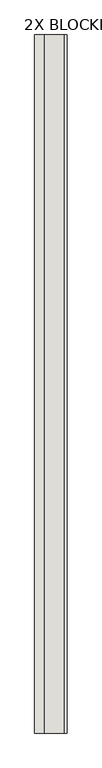
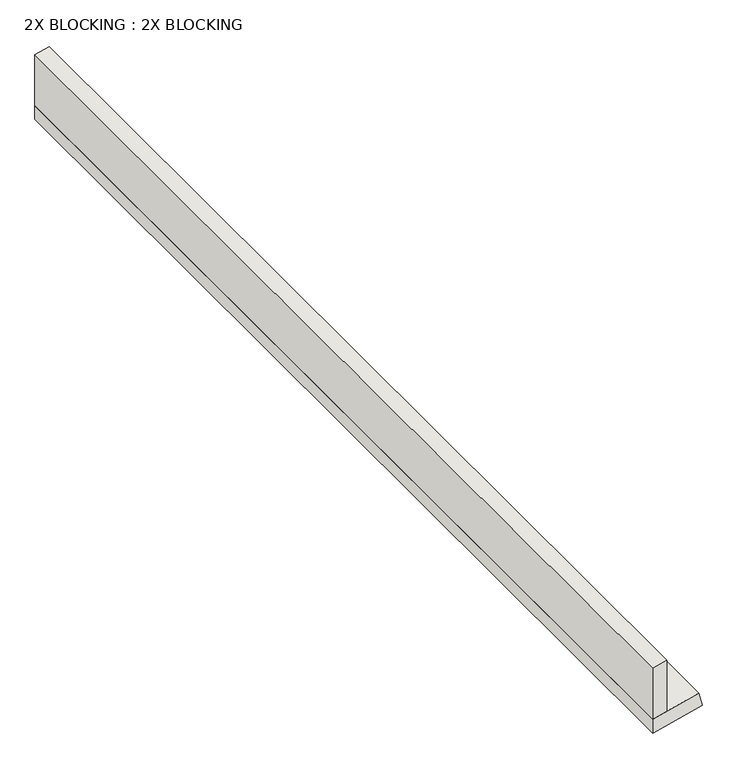
"""IFC4 building model written with IfcOpenShell, lengths in millimetres: wall geometry, 2X BLOCKING : 2X BLOCKING."""

import ifcopenshell
import ifcopenshell.guid

model = None  # the IFC model being written
_history = None  # IfcOwnerHistory: only IFC2X3 demands one
_inside = {}  # id of a spatial element -> (the spatial element, [elements in it])
_under = {}  # id of a project, library or spatial element -> (it, [spatial elements below it])
_declared = {}  # id of a project -> (the project, [libraries it declares])
_typed = {}  # id of a type object -> (the type object, [elements of that type])
_made_of = {}  # id of a material, layer set ... -> (it, [elements and type objects made of it])


def new_model(schema):
    """Start an empty IFC model of exactly this schema.

    Asked for "IFC4X3", IfcOpenShell would pick the latest addendum, in which some entities
    have other attributes; the version numbers below select the first issue.
    IFC2X3 requires an IfcOwnerHistory on every rooted entity: one is made here for all.
    """
    global model, _history
    if schema == "IFC4X3":
        model = ifcopenshell.file(schema_version=(4, 3, 0, 0))
    else:
        model = ifcopenshell.file(schema=schema)
    _inside.clear()
    _under.clear()
    _declared.clear()
    _typed.clear()
    _made_of.clear()
    _history = None
    if model.schema == "IFC2X3":
        org = make("IfcOrganization", Name="unknown")
        user = make(
            "IfcPersonAndOrganization",
            ThePerson=make("IfcPerson", FamilyName="unknown"),
            TheOrganization=org,
        )
        app = make(
            "IfcApplication",
            ApplicationDeveloper=org,
            Version="unknown",
            ApplicationFullName="unknown",
            ApplicationIdentifier="unknown",
        )
        _history = make(
            "IfcOwnerHistory",
            OwningUser=user,
            OwningApplication=app,
            ChangeAction="ADDED",
            CreationDate=0,
        )
    return model


def make(cls, **values):
    """One entity of the class cls with the attributes given. An attribute that is None is left unset."""
    return model.create_entity(
        cls, **{name: value for name, value in values.items() if value is not None}
    )


def rooted(cls, **values):
    """An entity with a GlobalId (a new one), such as an element, a storey or a relation."""
    return make(cls, GlobalId=ifcopenshell.guid.new(), OwnerHistory=_history, **values)


def si_unit(unit_type, name, prefix=None):
    """IfcSIUnit, for example si_unit("LENGTHUNIT", "METRE", prefix="MILLI")."""
    return make("IfcSIUnit", UnitType=unit_type, Prefix=prefix, Name=name)


def assignment(units):
    """IfcUnitAssignment: the units of a project."""
    return None if units is None else make("IfcUnitAssignment", Units=units)


def point(xyz):
    """IfcCartesianPoint."""
    return None if xyz is None else make("IfcCartesianPoint", Coordinates=xyz)


def direction(xyz):
    """IfcDirection."""
    return None if xyz is None else make("IfcDirection", DirectionRatios=xyz)


def frame(location, z_axis=None, x_axis=None):
    """IfcAxis2Placement3D, a coordinate frame: its origin and axes. An axis left out is left unset."""
    return make(
        "IfcAxis2Placement3D",
        Location=point(location),
        Axis=direction(z_axis),
        RefDirection=direction(x_axis),
    )


def origin():
    """The frame at (0, 0, 0) with its axes left unset."""
    return frame((0.0, 0.0, 0.0))


def place(relative_to, where):
    """IfcLocalPlacement: puts the frame where relative to a parent placement (None: the world)."""
    return make(
        "IfcLocalPlacement", PlacementRelTo=relative_to, RelativePlacement=where
    )


def context(
    kind, dimensions, precision=None, world=None, true_north=None, identifier=None
):
    """IfcGeometricRepresentationContext, for example the 3D "Model" context."""
    return make(
        "IfcGeometricRepresentationContext",
        ContextIdentifier=identifier,
        ContextType=kind,
        CoordinateSpaceDimension=dimensions,
        Precision=precision,
        WorldCoordinateSystem=world,
        TrueNorth=true_north,
    )


def project(units=None, contexts=None):
    """IfcProject with its units and contexts."""
    return rooted(
        "IfcProject",
        Name="project",
        RepresentationContexts=contexts,
        UnitsInContext=assignment(units),
    )


def spatial(cls, under=None, at=None, **own):
    """A site, building, storey or space (cls), placed at a placement, below another one or the project."""
    s = rooted(cls, ObjectPlacement=at, **own)
    if under is not None:
        _under.setdefault(under.id(), (under, []))[1].append(s)
    return s


def polyline(points):
    """IfcPolyline through the points."""
    return make("IfcPolyline", Points=[point(p) for p in points])


def outline(outer, holes=None, kind="AREA"):
    """IfcArbitraryClosedProfileDef: a profile drawn as a closed curve; with holes, ...WithVoids."""
    if holes is None:
        return make("IfcArbitraryClosedProfileDef", ProfileType=kind, OuterCurve=outer)
    return make(
        "IfcArbitraryProfileDefWithVoids",
        ProfileType=kind,
        OuterCurve=outer,
        InnerCurves=holes,
    )


def extrude(swept, where, along, depth):
    """IfcExtrudedAreaSolid: the profile swept, set in the frame where, extruded along a direction by depth."""
    return make(
        "IfcExtrudedAreaSolid",
        SweptArea=swept,
        Position=where,
        ExtrudedDirection=direction(along),
        Depth=depth,
    )


def shape(context_of_items, identifier, shape_type, items):
    """IfcShapeRepresentation: the items that make up one representation, for example the "Body"."""
    return make(
        "IfcShapeRepresentation",
        ContextOfItems=context_of_items,
        RepresentationIdentifier=identifier,
        RepresentationType=shape_type,
        Items=items,
    )


def source(mapping_origin, context_of_items, identifier, shape_type, items):
    """IfcRepresentationMap: a shape defined once, which mapped items show again and again."""
    return make(
        "IfcRepresentationMap",
        MappingOrigin=mapping_origin,
        MappedRepresentation=shape(context_of_items, identifier, shape_type, items),
    )


def transform(
    local_origin,
    x_axis=None,
    y_axis=None,
    z_axis=None,
    scale=None,
    scale2=None,
    scale3=None,
    uniform=True,
):
    """IfcCartesianTransformationOperator3D, or its non-uniform kind. x_axis, y_axis, z_axis: its Axis1, 2, 3."""
    if uniform:
        return make(
            "IfcCartesianTransformationOperator3D",
            Axis1=direction(x_axis),
            Axis2=direction(y_axis),
            LocalOrigin=point(local_origin),
            Scale=scale,
            Axis3=direction(z_axis),
        )
    return make(
        "IfcCartesianTransformationOperator3DnonUniform",
        Axis1=direction(x_axis),
        Axis2=direction(y_axis),
        LocalOrigin=point(local_origin),
        Scale=scale,
        Axis3=direction(z_axis),
        Scale2=scale2,
        Scale3=scale3,
    )


def mapped(mapping_source, mapping_target):
    """IfcMappedItem: shows the shape of a source again, moved by a transform."""
    return make(
        "IfcMappedItem", MappingSource=mapping_source, MappingTarget=mapping_target
    )


def made_of(thing, what):
    """Note that an element or type object is made of a material, layer set ...; save() writes the relation."""
    if what is not None:
        _made_of.setdefault(what.id(), (what, []))[1].append(thing)
    return thing


def element(
    cls,
    number,
    at=None,
    inside=None,
    cuts=None,
    type_object=None,
    material=None,
    context=None,
    identifier="Body",
    shape_type=None,
    held_by="IfcProductDefinitionShape",
    body=None,
    shapes=None,
    **own,
):
    """One element of the class cls, such as IfcWall. Its Tag is "e" and its number.

    at: its placement. inside: the storey or other place that contains it. cuts: it is an
    opening in that element (IfcRelVoidsElement). A single representation is given by context,
    identifier, shape_type and body (its items); several are given by shapes. held_by: the class
    of the entity that holds the representations. save() writes the other relations.
    """
    e = rooted(cls, Tag="e%d" % number, ObjectPlacement=at, **own)
    if body is not None:
        shapes = [shape(context, identifier, shape_type, body)]
    if shapes is not None:
        e.Representation = make(held_by, Representations=shapes)
    if inside is not None:
        _inside.setdefault(inside.id(), (inside, []))[1].append(e)
    if cuts is not None:
        rooted(
            "IfcRelVoidsElement", RelatingBuildingElement=cuts, RelatedOpeningElement=e
        )
    if type_object is not None:
        _typed.setdefault(type_object.id(), (type_object, []))[1].append(e)
    return made_of(e, material)


def aggregate(whole, parts):
    """IfcRelAggregates: a whole, such as a stair, and the parts it consists of."""
    return rooted("IfcRelAggregates", RelatingObject=whole, RelatedObjects=parts)


def save(model, path):
    """Write the relations noted so far, then the file.

    IfcRelAggregates (storeys below a building ...), IfcRelContainedInSpatialStructure (elements
    in a storey), IfcRelDefinesByType, IfcRelAssociatesMaterial and IfcRelDeclares: one each for
    every whole, place, type object, material and project.
    """
    for whole, parts in _under.values():
        aggregate(whole, parts)
    for where, things in _inside.values():
        rooted(
            "IfcRelContainedInSpatialStructure",
            RelatedElements=things,
            RelatingStructure=where,
        )
    for kind, things in _typed.values():
        rooted("IfcRelDefinesByType", RelatedObjects=things, RelatingType=kind)
    for what, things in _made_of.values():
        rooted("IfcRelAssociatesMaterial", RelatedObjects=things, RelatingMaterial=what)
    for by, libraries in _declared.values():
        rooted("IfcRelDeclares", RelatingContext=by, RelatedDefinitions=libraries)
    model.write(path)


def wall_2x_blocking_2x_blocking_4d35bf6a(model_context):
    return source(origin(), model_context, "Body", "SweptSolid", [
        extrude(outline(polyline([(2378.0799446, 17971.2961644), (2522.0767538, 17971.2961644), (2512.549464, 17933.1870052), (2368.55, 17933.1870052), (2378.0799446, 17971.2961644)])), frame((0.0, -3415.0384634, 0.0), z_axis=(0.0, 1.0, 0.0), x_axis=(0.0, 0.0, 1.0)), (0.0, 0.0, 1.0), 2862.7206389),
        extrude(outline(polyline([(2329.2673338, 17933.1870052), (2362.3499156, 18065.4804684), (2399.3206245, 18056.2352157), (2368.55, 17933.1870052), (2329.2673338, 17933.1870052)])), frame((0.0, -3415.0384634, 0.0), z_axis=(0.0, 1.0, 0.0), x_axis=(0.0, 0.0, 1.0)), (0.0, 0.0, 1.0), 2862.7206389),
    ])


if __name__ == "__main__":
    model = new_model("IFC4")
    model_context = context("Model", 3, world=origin())
    ifc_project = project(units=[si_unit("LENGTHUNIT", "METRE", prefix="MILLI")], contexts=[model_context])
    site = spatial("IfcSite", under=ifc_project)
    building = spatial("IfcBuilding", under=site)
    placement = place(None, origin())
    wall_2x_blocking_2x_blocking_shape = wall_2x_blocking_2x_blocking_4d35bf6a(model_context)
    element("IfcWall", 1, ObjectType="2X BLOCKING : 2X BLOCKING", at=placement, inside=building, context=model_context, shape_type="MappedRepresentation", body=[
        mapped(wall_2x_blocking_2x_blocking_shape, transform((0.0, 0.0, 0.0), x_axis=(1.0, 0.0, 0.0), y_axis=(0.0, 1.0, 0.0), z_axis=(0.0, 0.0, 1.0))),
    ])
    save(model, "model.ifc")

# Revit data of these elements
# Type "2X BLOCKING : 2X BLOCKING"
#   Structural Material = 2 X BLOCKING
# Element 1 (IfcWall, "2X BLOCKING : 2X BLOCKING")
#   Materials on its faces: "BLOCKING AS NEEDED"
# Materials
#   "2 X BLOCKING": class "Wood", colour RGB 234 198 147, transparency 0, Description = "Pinus Echinata", Cost = 0
#   "BLOCKING AS NEEDED": class "Wood", colour RGB 234 198 147, transparency 0, Description = "Pinus Echinata", Cost = 0
